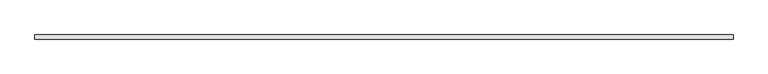
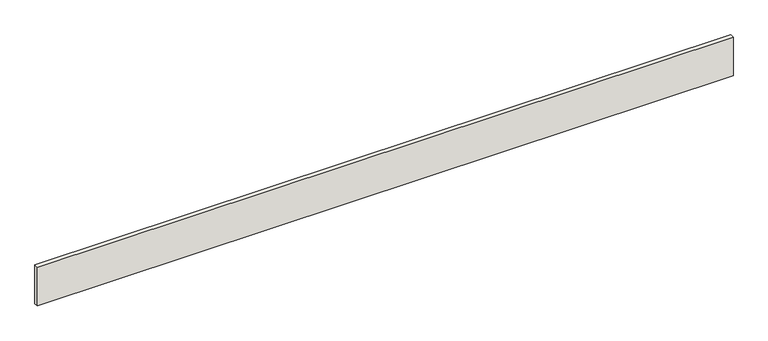
"""IFC4 building model written with IfcOpenShell, lengths in millimetres: wall geometry, Holzwand."""

from ifc_helpers import new_model, si_unit, origin, origin_with_axes, place, context, project, spatial, polyline, outline, extrude, source, transform, mapped, element, save


def wall_119e3faa(model_context):
    return source(origin(), model_context, "Body", "SweptSolid", [
        extrude(outline(polyline([(17000.0, 100.0), (17000.0, 0.0), (0.0, 0.0), (0.0, 100.0), (17000.0, 100.0)])), origin_with_axes(), (0.0, 0.0, 1.0), 1000.0),
    ])


if __name__ == "__main__":
    model = new_model("IFC4")
    model_context = context("Model", 3, world=origin())
    ifc_project = project(units=[si_unit("LENGTHUNIT", "METRE", prefix="MILLI")], contexts=[model_context])
    site = spatial("IfcSite", under=ifc_project)
    building = spatial("IfcBuilding", under=site)
    placement = place(None, origin())
    wall_shape = wall_119e3faa(model_context)
    element("IfcWall", 1, ObjectType="Holzwand", at=placement, inside=building, context=model_context, shape_type="MappedRepresentation", body=[
        mapped(wall_shape, transform((0.0, 0.0, 0.0), x_axis=(1.0, 0.0, 0.0), y_axis=(0.0, 1.0, 0.0), z_axis=(0.0, 0.0, 1.0))),
    ])
    save(model, "model.ifc")

# Revit data of these elements
# Element 1 (IfcWall, "Holzwand")
#   Materials on its faces: "glas"
# Materials
#   "glas": class "Unassigned", colour RGB 250 253 254, transparency 0.95
